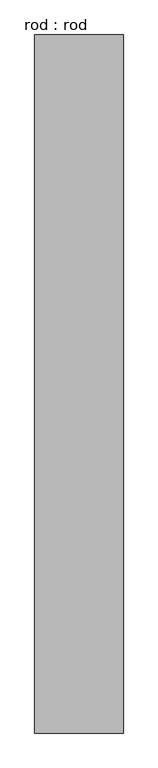
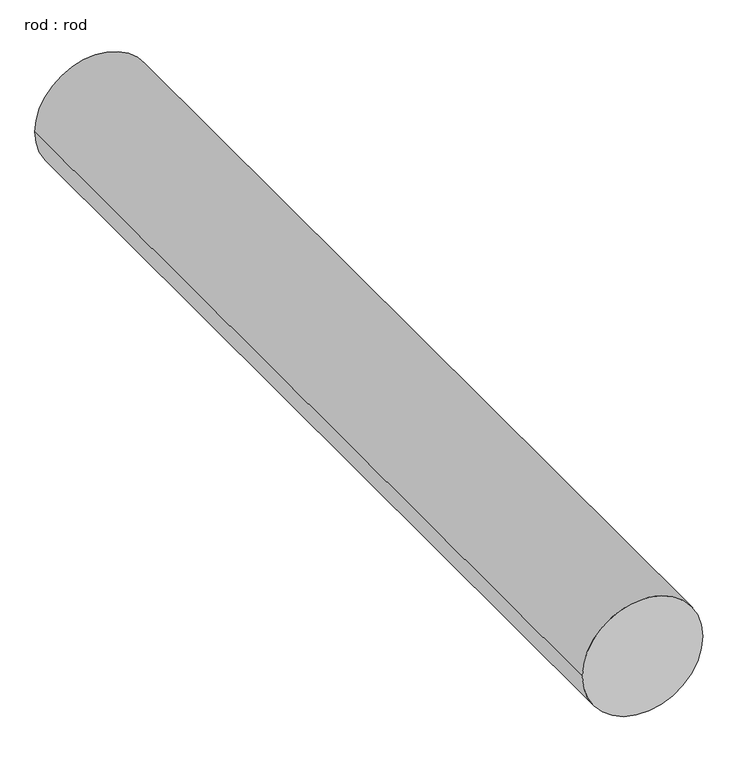
"""IFC4 building model written with IfcOpenShell, lengths in millimetres: proxy geometry, rod : rod."""

from ifc_helpers import new_model, si_unit, point, frame, frame_2d, origin, place, context, project, spatial, circle_curve, trimmed, segment, composite_curve, outline, extrude, source, transform, mapped, element, save


def rod_rod_3a2ab96c(model_context):
    return source(origin(), model_context, "Body", "SweptSolid", [
        extrude(outline(composite_curve([segment(trimmed(circle_curve(frame_2d((0.0108462, 0.0)), 200.0), [point((0.0108462, 200.0))], [point((0.0108462, -200.0))], False, "CARTESIAN"), True, "CONTINUOUS"), segment(trimmed(circle_curve(frame_2d((0.0108462, 0.0)), 200.0), [point((0.0108462, -200.0))], [point((0.0108462, 200.0))], False, "CARTESIAN"), True, "CONTINUOUS")], self_intersect=False)), frame((0.0, 2517.7286153, 0.0), z_axis=(0.0, 1.0, 0.0), x_axis=(0.0, 0.0, 1.0)), (0.0, 0.0, 1.0), 3150.0),
    ])


if __name__ == "__main__":
    model = new_model("IFC4")
    model_context = context("Model", 3, world=origin())
    ifc_project = project(units=[si_unit("LENGTHUNIT", "METRE", prefix="MILLI")], contexts=[model_context])
    site = spatial("IfcSite", under=ifc_project)
    building = spatial("IfcBuilding", under=site)
    placement = place(None, origin())
    rod_rod_shape = rod_rod_3a2ab96c(model_context)
    element("IfcBuildingElementProxy", 1, Name="rod : rod", ObjectType="rod : rod", at=placement, inside=building, context=model_context, shape_type="MappedRepresentation", body=[
        mapped(rod_rod_shape, transform((0.0, 0.0, 0.0), x_axis=(1.0, 0.0, 0.0), y_axis=(0.0, 1.0, 0.0), z_axis=(0.0, 0.0, 1.0))),
    ])
    save(model, "model.ifc")

# Revit data of these elements
# Type "rod : rod"
#   Default Elevation = 0
